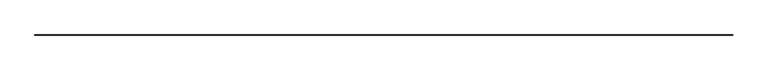
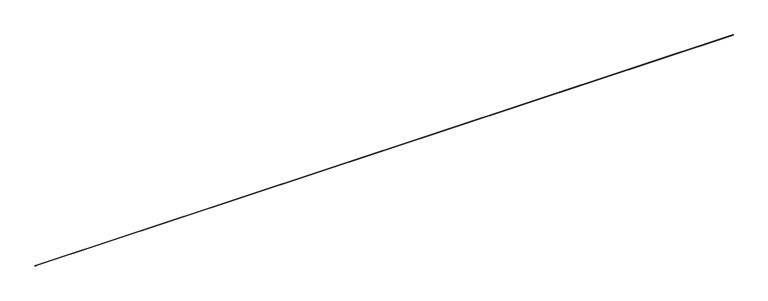
"""IFC4 building model written with IfcOpenShell, lengths in millimetres: proxy geometry, Generic Models 7:Generic Models 1:1:Generic Models 1:1 : Generic Models 7:Generic Models 1:337419:56 : Generic Models 7:Generic Models 1:1:Generic Models 1:1 : Generic Models 7:Generic Models 1:337419:306201."""

import ifcopenshell
import ifcopenshell.guid

model = None  # the IFC model being written
_history = None  # IfcOwnerHistory: only IFC2X3 demands one
_inside = {}  # id of a spatial element -> (the spatial element, [elements in it])
_under = {}  # id of a project, library or spatial element -> (it, [spatial elements below it])
_declared = {}  # id of a project -> (the project, [libraries it declares])
_typed = {}  # id of a type object -> (the type object, [elements of that type])
_made_of = {}  # id of a material, layer set ... -> (it, [elements and type objects made of it])


def new_model(schema):
    """Start an empty IFC model of exactly this schema.

    Asked for "IFC4X3", IfcOpenShell would pick the latest addendum, in which some entities
    have other attributes; the version numbers below select the first issue.
    IFC2X3 requires an IfcOwnerHistory on every rooted entity: one is made here for all.
    """
    global model, _history
    if schema == "IFC4X3":
        model = ifcopenshell.file(schema_version=(4, 3, 0, 0))
    else:
        model = ifcopenshell.file(schema=schema)
    _inside.clear()
    _under.clear()
    _declared.clear()
    _typed.clear()
    _made_of.clear()
    _history = None
    if model.schema == "IFC2X3":
        org = make("IfcOrganization", Name="unknown")
        user = make(
            "IfcPersonAndOrganization",
            ThePerson=make("IfcPerson", FamilyName="unknown"),
            TheOrganization=org,
        )
        app = make(
            "IfcApplication",
            ApplicationDeveloper=org,
            Version="unknown",
            ApplicationFullName="unknown",
            ApplicationIdentifier="unknown",
        )
        _history = make(
            "IfcOwnerHistory",
            OwningUser=user,
            OwningApplication=app,
            ChangeAction="ADDED",
            CreationDate=0,
        )
    return model


def make(cls, **values):
    """One entity of the class cls with the attributes given. An attribute that is None is left unset."""
    return model.create_entity(
        cls, **{name: value for name, value in values.items() if value is not None}
    )


def rooted(cls, **values):
    """An entity with a GlobalId (a new one), such as an element, a storey or a relation."""
    return make(cls, GlobalId=ifcopenshell.guid.new(), OwnerHistory=_history, **values)


def si_unit(unit_type, name, prefix=None):
    """IfcSIUnit, for example si_unit("LENGTHUNIT", "METRE", prefix="MILLI")."""
    return make("IfcSIUnit", UnitType=unit_type, Prefix=prefix, Name=name)


def assignment(units):
    """IfcUnitAssignment: the units of a project."""
    return None if units is None else make("IfcUnitAssignment", Units=units)


def point(xyz):
    """IfcCartesianPoint."""
    return None if xyz is None else make("IfcCartesianPoint", Coordinates=xyz)


def direction(xyz):
    """IfcDirection."""
    return None if xyz is None else make("IfcDirection", DirectionRatios=xyz)


def frame(location, z_axis=None, x_axis=None):
    """IfcAxis2Placement3D, a coordinate frame: its origin and axes. An axis left out is left unset."""
    return make(
        "IfcAxis2Placement3D",
        Location=point(location),
        Axis=direction(z_axis),
        RefDirection=direction(x_axis),
    )


def origin():
    """The frame at (0, 0, 0) with its axes left unset."""
    return frame((0.0, 0.0, 0.0))


def place(relative_to, where):
    """IfcLocalPlacement: puts the frame where relative to a parent placement (None: the world)."""
    return make(
        "IfcLocalPlacement", PlacementRelTo=relative_to, RelativePlacement=where
    )


def context(
    kind, dimensions, precision=None, world=None, true_north=None, identifier=None
):
    """IfcGeometricRepresentationContext, for example the 3D "Model" context."""
    return make(
        "IfcGeometricRepresentationContext",
        ContextIdentifier=identifier,
        ContextType=kind,
        CoordinateSpaceDimension=dimensions,
        Precision=precision,
        WorldCoordinateSystem=world,
        TrueNorth=true_north,
    )


def project(units=None, contexts=None):
    """IfcProject with its units and contexts."""
    return rooted(
        "IfcProject",
        Name="project",
        RepresentationContexts=contexts,
        UnitsInContext=assignment(units),
    )


def spatial(cls, under=None, at=None, **own):
    """A site, building, storey or space (cls), placed at a placement, below another one or the project."""
    s = rooted(cls, ObjectPlacement=at, **own)
    if under is not None:
        _under.setdefault(under.id(), (under, []))[1].append(s)
    return s


def polyline(points):
    """IfcPolyline through the points."""
    return make("IfcPolyline", Points=[point(p) for p in points])


def outline(outer, holes=None, kind="AREA"):
    """IfcArbitraryClosedProfileDef: a profile drawn as a closed curve; with holes, ...WithVoids."""
    if holes is None:
        return make("IfcArbitraryClosedProfileDef", ProfileType=kind, OuterCurve=outer)
    return make(
        "IfcArbitraryProfileDefWithVoids",
        ProfileType=kind,
        OuterCurve=outer,
        InnerCurves=holes,
    )


def extrude(swept, where, along, depth):
    """IfcExtrudedAreaSolid: the profile swept, set in the frame where, extruded along a direction by depth."""
    return make(
        "IfcExtrudedAreaSolid",
        SweptArea=swept,
        Position=where,
        ExtrudedDirection=direction(along),
        Depth=depth,
    )


def shape(context_of_items, identifier, shape_type, items):
    """IfcShapeRepresentation: the items that make up one representation, for example the "Body"."""
    return make(
        "IfcShapeRepresentation",
        ContextOfItems=context_of_items,
        RepresentationIdentifier=identifier,
        RepresentationType=shape_type,
        Items=items,
    )


def source(mapping_origin, context_of_items, identifier, shape_type, items):
    """IfcRepresentationMap: a shape defined once, which mapped items show again and again."""
    return make(
        "IfcRepresentationMap",
        MappingOrigin=mapping_origin,
        MappedRepresentation=shape(context_of_items, identifier, shape_type, items),
    )


def transform(
    local_origin,
    x_axis=None,
    y_axis=None,
    z_axis=None,
    scale=None,
    scale2=None,
    scale3=None,
    uniform=True,
):
    """IfcCartesianTransformationOperator3D, or its non-uniform kind. x_axis, y_axis, z_axis: its Axis1, 2, 3."""
    if uniform:
        return make(
            "IfcCartesianTransformationOperator3D",
            Axis1=direction(x_axis),
            Axis2=direction(y_axis),
            LocalOrigin=point(local_origin),
            Scale=scale,
            Axis3=direction(z_axis),
        )
    return make(
        "IfcCartesianTransformationOperator3DnonUniform",
        Axis1=direction(x_axis),
        Axis2=direction(y_axis),
        LocalOrigin=point(local_origin),
        Scale=scale,
        Axis3=direction(z_axis),
        Scale2=scale2,
        Scale3=scale3,
    )


def mapped(mapping_source, mapping_target):
    """IfcMappedItem: shows the shape of a source again, moved by a transform."""
    return make(
        "IfcMappedItem", MappingSource=mapping_source, MappingTarget=mapping_target
    )


def made_of(thing, what):
    """Note that an element or type object is made of a material, layer set ...; save() writes the relation."""
    if what is not None:
        _made_of.setdefault(what.id(), (what, []))[1].append(thing)
    return thing


def element(
    cls,
    number,
    at=None,
    inside=None,
    cuts=None,
    type_object=None,
    material=None,
    context=None,
    identifier="Body",
    shape_type=None,
    held_by="IfcProductDefinitionShape",
    body=None,
    shapes=None,
    **own,
):
    """One element of the class cls, such as IfcWall. Its Tag is "e" and its number.

    at: its placement. inside: the storey or other place that contains it. cuts: it is an
    opening in that element (IfcRelVoidsElement). A single representation is given by context,
    identifier, shape_type and body (its items); several are given by shapes. held_by: the class
    of the entity that holds the representations. save() writes the other relations.
    """
    e = rooted(cls, Tag="e%d" % number, ObjectPlacement=at, **own)
    if body is not None:
        shapes = [shape(context, identifier, shape_type, body)]
    if shapes is not None:
        e.Representation = make(held_by, Representations=shapes)
    if inside is not None:
        _inside.setdefault(inside.id(), (inside, []))[1].append(e)
    if cuts is not None:
        rooted(
            "IfcRelVoidsElement", RelatingBuildingElement=cuts, RelatedOpeningElement=e
        )
    if type_object is not None:
        _typed.setdefault(type_object.id(), (type_object, []))[1].append(e)
    return made_of(e, material)


def aggregate(whole, parts):
    """IfcRelAggregates: a whole, such as a stair, and the parts it consists of."""
    return rooted("IfcRelAggregates", RelatingObject=whole, RelatedObjects=parts)


def save(model, path):
    """Write the relations noted so far, then the file.

    IfcRelAggregates (storeys below a building ...), IfcRelContainedInSpatialStructure (elements
    in a storey), IfcRelDefinesByType, IfcRelAssociatesMaterial and IfcRelDeclares: one each for
    every whole, place, type object, material and project.
    """
    for whole, parts in _under.values():
        aggregate(whole, parts)
    for where, things in _inside.values():
        rooted(
            "IfcRelContainedInSpatialStructure",
            RelatedElements=things,
            RelatingStructure=where,
        )
    for kind, things in _typed.values():
        rooted("IfcRelDefinesByType", RelatedObjects=things, RelatingType=kind)
    for what, things in _made_of.values():
        rooted("IfcRelAssociatesMaterial", RelatedObjects=things, RelatingMaterial=what)
    for by, libraries in _declared.values():
        rooted("IfcRelDeclares", RelatingContext=by, RelatedDefinitions=libraries)
    model.write(path)


def generic_models_9fc63045(model_context):
    return source(origin(), model_context, "Body", "SweptSolid", [
        extrude(outline(polyline([(-578859.6152195, 4.5309106), (-578860.9558801, 3.4217064), (-578861.408944, 2.4027259), (-578861.2559077, 1.3418402), (-578860.5207124, 0.405015), (-578859.5534942, -0.130913), (-578868.4086871, -0.130913), (-578868.0869737, 2.1348593), (-578868.3237006, 3.802086), (-578868.6085165, 4.5309106), (-578859.6152195, 4.5309106)])), frame((557809.7867239, 0.0, 0.0), z_axis=(1.0, 0.0, 0.0), x_axis=(0.0, 1.0, 0.0)), (0.0, 0.0, 1.0), 38252.9096551),
    ])


if __name__ == "__main__":
    model = new_model("IFC4")
    model_context = context("Model", 3, world=origin())
    ifc_project = project(units=[si_unit("LENGTHUNIT", "METRE", prefix="MILLI")], contexts=[model_context])
    site = spatial("IfcSite", under=ifc_project)
    building = spatial("IfcBuilding", under=site)
    placement = place(None, origin())
    generic_models_shape = generic_models_9fc63045(model_context)
    element("IfcBuildingElementProxy", 1, Name="Generic Models 7:Generic Models 1:1:Generic Models 1:1 : Generic Models 7:Generic Models 1:337419:56 : Generic Models 7:Generic Models 1:1:Generic Models 1:1 : Generic Models 7:Generic Models 1:337419:306201", ObjectType="Generic Models 7:Generic Models 1:1:Generic Models 1:1 : Generic Models 7:Generic Models 1:337419:56 : Generic Models 7:Generic Models 1:1:Generic Models 1:1 : Generic Models 7:Generic Models 1:337419:306201", at=placement, inside=building, context=model_context, shape_type="MappedRepresentation", body=[
        mapped(generic_models_shape, transform((0.0, 0.0, 0.0), x_axis=(1.0, 0.0, 0.0), y_axis=(0.0, 1.0, 0.0), z_axis=(0.0, 0.0, 1.0))),
    ])
    save(model, "model.ifc")

# Revit data of these elements
# Type "Generic Models 7:Generic Models 1:1:Generic Models 1:1 : Generic Models 7:Generic Models 1:337419:56 : Generic Models 7:Generic Models 1:1:Generic Models 1:1 : Generic Models 7:Generic Models 1:337419:306201"
#   NameOverride = "Generic Models 7:Generic Models 1:1:Generic Models 1:1 : Generic Models 7:Generic Models 1:337419:306201"
#   ObjectTypeOverride = "Generic Models 1:1 : Generic Models 7:Generic Models 1:337419"
#   Reference = "Generic Models 1"
#   Tag = "306201"
# Element 1 (IfcBuildingElementProxy, "Generic Models 7:Generic Models 1:1:Generic Models 1:1 : Generic Models 7:Generic Models 1:337419:56 : Generic Models 7:Generic Models 1:1:Generic Models 1:1 : Generic Models 7:Generic Models 1:337419:306201")
#   Materials on its faces: "SEMI-RIGID EPOXY SEALANT W/ BACKROD (REMOVE TEMP. JOINT FORM)"
# Materials
#   "SEMI-RIGID EPOXY SEALANT W/ BACKROD (REMOVE TEMP. JOINT FORM)": class "Unassigned", colour RGB 120 120 120, transparency 0, Cost = 0
